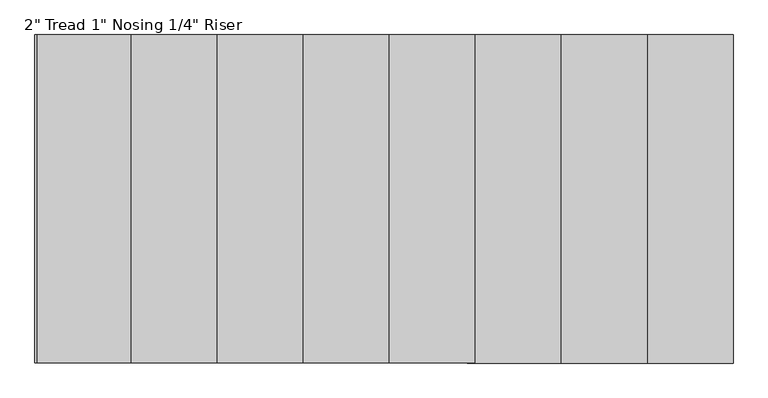
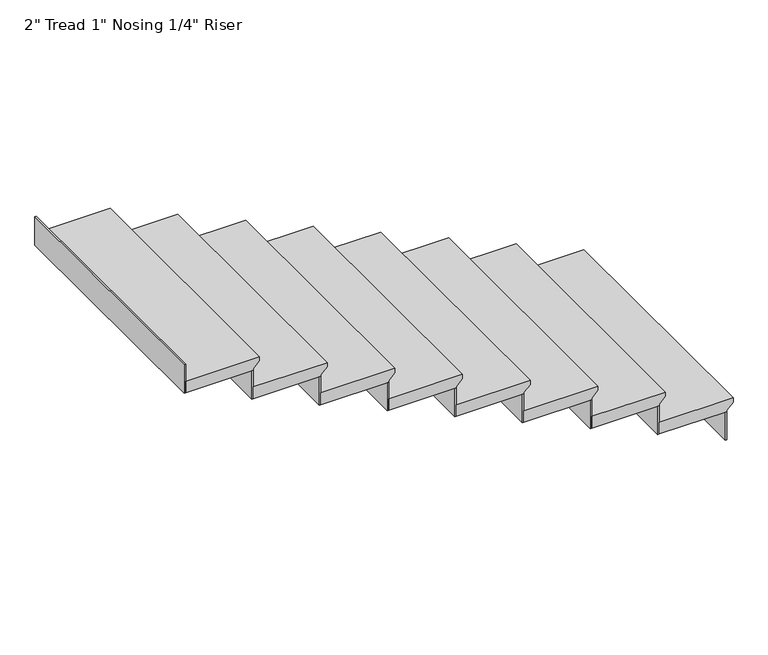
"""IFC4 building model written with IfcOpenShell, lengths in millimetres: stair flight geometry."""

import ifcopenshell
import ifcopenshell.guid

model = None  # the IFC model being written
_history = None  # IfcOwnerHistory: only IFC2X3 demands one
_inside = {}  # id of a spatial element -> (the spatial element, [elements in it])
_under = {}  # id of a project, library or spatial element -> (it, [spatial elements below it])
_declared = {}  # id of a project -> (the project, [libraries it declares])
_typed = {}  # id of a type object -> (the type object, [elements of that type])
_made_of = {}  # id of a material, layer set ... -> (it, [elements and type objects made of it])


def new_model(schema):
    """Start an empty IFC model of exactly this schema.

    Asked for "IFC4X3", IfcOpenShell would pick the latest addendum, in which some entities
    have other attributes; the version numbers below select the first issue.
    IFC2X3 requires an IfcOwnerHistory on every rooted entity: one is made here for all.
    """
    global model, _history
    if schema == "IFC4X3":
        model = ifcopenshell.file(schema_version=(4, 3, 0, 0))
    else:
        model = ifcopenshell.file(schema=schema)
    _inside.clear()
    _under.clear()
    _declared.clear()
    _typed.clear()
    _made_of.clear()
    _history = None
    if model.schema == "IFC2X3":
        org = make("IfcOrganization", Name="unknown")
        user = make(
            "IfcPersonAndOrganization",
            ThePerson=make("IfcPerson", FamilyName="unknown"),
            TheOrganization=org,
        )
        app = make(
            "IfcApplication",
            ApplicationDeveloper=org,
            Version="unknown",
            ApplicationFullName="unknown",
            ApplicationIdentifier="unknown",
        )
        _history = make(
            "IfcOwnerHistory",
            OwningUser=user,
            OwningApplication=app,
            ChangeAction="ADDED",
            CreationDate=0,
        )
    return model


def make(cls, **values):
    """One entity of the class cls with the attributes given. An attribute that is None is left unset."""
    return model.create_entity(
        cls, **{name: value for name, value in values.items() if value is not None}
    )


def rooted(cls, **values):
    """An entity with a GlobalId (a new one), such as an element, a storey or a relation."""
    return make(cls, GlobalId=ifcopenshell.guid.new(), OwnerHistory=_history, **values)


def si_unit(unit_type, name, prefix=None):
    """IfcSIUnit, for example si_unit("LENGTHUNIT", "METRE", prefix="MILLI")."""
    return make("IfcSIUnit", UnitType=unit_type, Prefix=prefix, Name=name)


def assignment(units):
    """IfcUnitAssignment: the units of a project."""
    return None if units is None else make("IfcUnitAssignment", Units=units)


def point(xyz):
    """IfcCartesianPoint."""
    return None if xyz is None else make("IfcCartesianPoint", Coordinates=xyz)


def direction(xyz):
    """IfcDirection."""
    return None if xyz is None else make("IfcDirection", DirectionRatios=xyz)


def frame(location, z_axis=None, x_axis=None):
    """IfcAxis2Placement3D, a coordinate frame: its origin and axes. An axis left out is left unset."""
    return make(
        "IfcAxis2Placement3D",
        Location=point(location),
        Axis=direction(z_axis),
        RefDirection=direction(x_axis),
    )


def origin():
    """The frame at (0, 0, 0) with its axes left unset."""
    return frame((0.0, 0.0, 0.0))


def place(relative_to, where):
    """IfcLocalPlacement: puts the frame where relative to a parent placement (None: the world)."""
    return make(
        "IfcLocalPlacement", PlacementRelTo=relative_to, RelativePlacement=where
    )


def context(
    kind, dimensions, precision=None, world=None, true_north=None, identifier=None
):
    """IfcGeometricRepresentationContext, for example the 3D "Model" context."""
    return make(
        "IfcGeometricRepresentationContext",
        ContextIdentifier=identifier,
        ContextType=kind,
        CoordinateSpaceDimension=dimensions,
        Precision=precision,
        WorldCoordinateSystem=world,
        TrueNorth=true_north,
    )


def project(units=None, contexts=None):
    """IfcProject with its units and contexts."""
    return rooted(
        "IfcProject",
        Name="project",
        RepresentationContexts=contexts,
        UnitsInContext=assignment(units),
    )


def spatial(cls, under=None, at=None, **own):
    """A site, building, storey or space (cls), placed at a placement, below another one or the project."""
    s = rooted(cls, ObjectPlacement=at, **own)
    if under is not None:
        _under.setdefault(under.id(), (under, []))[1].append(s)
    return s


def faces_of(points, faces, orient=None, outer=None):
    """IfcFace entities. A face is a list of loops; a loop is a list of indices into points, from 0.

    orient and outer hold one flag for each loop. By default every Orientation is true, the
    first loop of a face is its IfcFaceOuterBound and the others are IfcFaceBound.
    """
    made = []
    for i, loops in enumerate(faces):
        bounds = []
        for j, loop in enumerate(loops):
            is_outer = j == 0 if outer is None else outer[i][j]
            bounds.append(
                make(
                    "IfcFaceOuterBound" if is_outer else "IfcFaceBound",
                    Bound=make("IfcPolyLoop", Polygon=[points[k] for k in loop]),
                    Orientation=True if orient is None else orient[i][j],
                )
            )
        made.append(make("IfcFace", Bounds=bounds))
    return made


def faceted_brep(points, faces, orient=None, outer=None, voids=None):
    """IfcFacetedBrep: a solid bounded by flat faces; with voids (closed shells), ...WithVoids."""
    shared = [point(p) for p in points]
    hull = make("IfcClosedShell", CfsFaces=faces_of(shared, faces, orient, outer))
    if voids is None:
        return make("IfcFacetedBrep", Outer=hull)
    return make(
        "IfcFacetedBrepWithVoids",
        Outer=hull,
        Voids=[
            make(cls, CfsFaces=faces_of(shared, fs, o, b)) for cls, fs, o, b in voids
        ],
    )


def shape(context_of_items, identifier, shape_type, items):
    """IfcShapeRepresentation: the items that make up one representation, for example the "Body"."""
    return make(
        "IfcShapeRepresentation",
        ContextOfItems=context_of_items,
        RepresentationIdentifier=identifier,
        RepresentationType=shape_type,
        Items=items,
    )


def source(mapping_origin, context_of_items, identifier, shape_type, items):
    """IfcRepresentationMap: a shape defined once, which mapped items show again and again."""
    return make(
        "IfcRepresentationMap",
        MappingOrigin=mapping_origin,
        MappedRepresentation=shape(context_of_items, identifier, shape_type, items),
    )


def transform(
    local_origin,
    x_axis=None,
    y_axis=None,
    z_axis=None,
    scale=None,
    scale2=None,
    scale3=None,
    uniform=True,
):
    """IfcCartesianTransformationOperator3D, or its non-uniform kind. x_axis, y_axis, z_axis: its Axis1, 2, 3."""
    if uniform:
        return make(
            "IfcCartesianTransformationOperator3D",
            Axis1=direction(x_axis),
            Axis2=direction(y_axis),
            LocalOrigin=point(local_origin),
            Scale=scale,
            Axis3=direction(z_axis),
        )
    return make(
        "IfcCartesianTransformationOperator3DnonUniform",
        Axis1=direction(x_axis),
        Axis2=direction(y_axis),
        LocalOrigin=point(local_origin),
        Scale=scale,
        Axis3=direction(z_axis),
        Scale2=scale2,
        Scale3=scale3,
    )


def mapped(mapping_source, mapping_target):
    """IfcMappedItem: shows the shape of a source again, moved by a transform."""
    return make(
        "IfcMappedItem", MappingSource=mapping_source, MappingTarget=mapping_target
    )


def made_of(thing, what):
    """Note that an element or type object is made of a material, layer set ...; save() writes the relation."""
    if what is not None:
        _made_of.setdefault(what.id(), (what, []))[1].append(thing)
    return thing


def element(
    cls,
    number,
    at=None,
    inside=None,
    cuts=None,
    type_object=None,
    material=None,
    context=None,
    identifier="Body",
    shape_type=None,
    held_by="IfcProductDefinitionShape",
    body=None,
    shapes=None,
    **own,
):
    """One element of the class cls, such as IfcWall. Its Tag is "e" and its number.

    at: its placement. inside: the storey or other place that contains it. cuts: it is an
    opening in that element (IfcRelVoidsElement). A single representation is given by context,
    identifier, shape_type and body (its items); several are given by shapes. held_by: the class
    of the entity that holds the representations. save() writes the other relations.
    """
    e = rooted(cls, Tag="e%d" % number, ObjectPlacement=at, **own)
    if body is not None:
        shapes = [shape(context, identifier, shape_type, body)]
    if shapes is not None:
        e.Representation = make(held_by, Representations=shapes)
    if inside is not None:
        _inside.setdefault(inside.id(), (inside, []))[1].append(e)
    if cuts is not None:
        rooted(
            "IfcRelVoidsElement", RelatingBuildingElement=cuts, RelatedOpeningElement=e
        )
    if type_object is not None:
        _typed.setdefault(type_object.id(), (type_object, []))[1].append(e)
    return made_of(e, material)


def aggregate(whole, parts):
    """IfcRelAggregates: a whole, such as a stair, and the parts it consists of."""
    return rooted("IfcRelAggregates", RelatingObject=whole, RelatedObjects=parts)


def save(model, path):
    """Write the relations noted so far, then the file.

    IfcRelAggregates (storeys below a building ...), IfcRelContainedInSpatialStructure (elements
    in a storey), IfcRelDefinesByType, IfcRelAssociatesMaterial and IfcRelDeclares: one each for
    every whole, place, type object, material and project.
    """
    for whole, parts in _under.values():
        aggregate(whole, parts)
    for where, things in _inside.values():
        rooted(
            "IfcRelContainedInSpatialStructure",
            RelatedElements=things,
            RelatingStructure=where,
        )
    for kind, things in _typed.values():
        rooted("IfcRelDefinesByType", RelatedObjects=things, RelatingType=kind)
    for what, things in _made_of.values():
        rooted("IfcRelAssociatesMaterial", RelatedObjects=things, RelatingMaterial=what)
    for by, libraries in _declared.values():
        rooted("IfcRelDeclares", RelatingContext=by, RelatedDefinitions=libraries)
    model.write(path)


def stair_flight_a08092b1(model_context):
    return source(origin(), model_context, "Body", "Brep", [
        faceted_brep([(665956.388677, -549416.0413841, 1216.6256757), (665956.388677, -549416.0413841, 1235.6756757), (665956.388677, -550482.8413841, 1235.6756757), (665956.388677, -550482.8413841, 1216.6256757), (665930.988677, -549416.0413841, 1191.2256757), (665930.988677, -550482.8413841, 1191.2256757), (665651.588677, -549416.0413841, 1235.6756757), (665651.588677, -550482.8413841, 1235.6756757), (665930.988677, -550482.8413841, 1184.8756757), (665651.588677, -550482.8413841, 1184.8756757), (665651.588677, -549416.0413841, 1184.8756757), (665930.988677, -549416.0413841, 1184.8756757)], [[[0, 1, 2, 3]], [[4, 0, 3, 5]], [[2, 1, 6, 7]], [[8, 9, 10, 11]], [[2, 7, 9, 8, 5, 3]], [[8, 11, 4, 5]], [[6, 1, 0, 4, 11, 10]], [[7, 6, 10, 9]]]),
        faceted_brep([(665930.988677, -549416.0413841, 1184.8756757), (665930.988677, -549416.0413841, 1061.3081081), (665924.638677, -549416.0413841, 1061.3081081), (665924.638677, -549416.0413841, 1184.8756757), (665930.988677, -550482.8413841, 1184.8756757), (665924.638677, -550482.8413841, 1184.8756757), (665924.638677, -550482.8413841, 1061.3081081), (665930.988677, -550482.8413841, 1061.3081081)], [[[0, 1, 2, 3]], [[4, 5, 6, 7]], [[1, 0, 4, 7]], [[2, 1, 7, 6]], [[3, 2, 6, 5]], [[0, 3, 5, 4]]]),
        faceted_brep([(665651.588677, -549416.0413841, 1308.4432432), (665651.588677, -549416.0413841, 1184.8756757), (665645.238677, -549416.0413841, 1184.8756757), (665645.238677, -549416.0413841, 1308.4432432), (665651.588677, -550482.8413841, 1308.4432432), (665645.238677, -550482.8413841, 1308.4432432), (665645.238677, -550482.8413841, 1184.8756757), (665651.588677, -550482.8413841, 1184.8756757)], [[[0, 1, 2, 3]], [[4, 5, 6, 7]], [[1, 0, 4, 7]], [[2, 1, 7, 6]], [[3, 2, 6, 5]], [[0, 3, 5, 4]]]),
        faceted_brep([(665676.988677, -550482.8413841, 1359.2432432), (665676.988677, -549416.0413841, 1359.2432432), (665372.188677, -549416.0413841, 1359.2432432), (665372.188677, -550482.8413841, 1359.2432432), (665651.588677, -550482.8413841, 1308.4432432), (665372.188677, -550482.8413841, 1308.4432432), (665372.188677, -549416.0413841, 1308.4432432), (665651.588677, -549416.0413841, 1308.4432432), (665651.588677, -550482.8413841, 1314.7932432), (665676.988677, -550482.8413841, 1340.1932432), (665651.588677, -549416.0413841, 1314.7932432), (665676.988677, -549416.0413841, 1340.1932432)], [[[0, 1, 2, 3]], [[4, 5, 6, 7]], [[0, 3, 5, 4, 8, 9]], [[4, 7, 10, 8]], [[2, 1, 11, 10, 7, 6]], [[3, 2, 6, 5]], [[11, 1, 0, 9]], [[10, 11, 9, 8]]]),
        faceted_brep([(665372.188677, -549416.0413841, 1432.0108108), (665372.188677, -549416.0413841, 1308.4432432), (665365.838677, -549416.0413841, 1308.4432432), (665365.838677, -549416.0413841, 1432.0108108), (665372.188677, -550482.8413841, 1432.0108108), (665365.838677, -550482.8413841, 1432.0108108), (665365.838677, -550482.8413841, 1308.4432432), (665372.188677, -550482.8413841, 1308.4432432)], [[[0, 1, 2, 3]], [[4, 5, 6, 7]], [[1, 0, 4, 7]], [[2, 1, 7, 6]], [[3, 2, 6, 5]], [[0, 3, 5, 4]]]),
        faceted_brep([(665397.588677, -550482.8413841, 1482.8108108), (665397.588677, -549416.0413841, 1482.8108108), (665092.788677, -549416.0413841, 1482.8108108), (665092.788677, -550482.8413841, 1482.8108108), (665372.188677, -550482.8413841, 1432.0108108), (665092.788677, -550482.8413841, 1432.0108108), (665092.788677, -549416.0413841, 1432.0108108), (665372.188677, -549416.0413841, 1432.0108108), (665372.188677, -550482.8413841, 1438.3608108), (665397.588677, -550482.8413841, 1463.7608108), (665372.188677, -549416.0413841, 1438.3608108), (665397.588677, -549416.0413841, 1463.7608108)], [[[0, 1, 2, 3]], [[4, 5, 6, 7]], [[0, 3, 5, 4, 8, 9]], [[4, 7, 10, 8]], [[2, 1, 11, 10, 7, 6]], [[3, 2, 6, 5]], [[11, 1, 0, 9]], [[10, 11, 9, 8]]]),
        faceted_brep([(665092.788677, -549416.0413841, 1555.5783784), (665092.788677, -549416.0413841, 1432.0108108), (665086.438677, -549416.0413841, 1432.0108108), (665086.438677, -549416.0413841, 1555.5783784), (665092.788677, -550482.8413841, 1555.5783784), (665086.438677, -550482.8413841, 1555.5783784), (665086.438677, -550482.8413841, 1432.0108108), (665092.788677, -550482.8413841, 1432.0108108)], [[[0, 1, 2, 3]], [[4, 5, 6, 7]], [[1, 0, 4, 7]], [[2, 1, 7, 6]], [[3, 2, 6, 5]], [[0, 3, 5, 4]]]),
        faceted_brep([(665118.188677, -550482.8413841, 1606.3783784), (665118.188677, -549416.0413841, 1606.3783784), (664813.388677, -549416.0413841, 1606.3783784), (664813.388677, -550482.8413841, 1606.3783784), (665092.788677, -550482.8413841, 1555.5783784), (664813.388677, -550482.8413841, 1555.5783784), (664813.388677, -549416.0413841, 1555.5783784), (665092.788677, -549416.0413841, 1555.5783784), (665092.788677, -550482.8413841, 1561.9283784), (665118.188677, -550482.8413841, 1587.3283784), (665092.788677, -549416.0413841, 1561.9283784), (665118.188677, -549416.0413841, 1587.3283784)], [[[0, 1, 2, 3]], [[4, 5, 6, 7]], [[0, 3, 5, 4, 8, 9]], [[4, 7, 10, 8]], [[2, 1, 11, 10, 7, 6]], [[3, 2, 6, 5]], [[11, 1, 0, 9]], [[10, 11, 9, 8]]]),
        faceted_brep([(664813.388677, -549416.0413841, 1679.1459459), (664813.388677, -549416.0413841, 1555.5783784), (664807.038677, -549416.0413841, 1555.5783784), (664807.038677, -549416.0413841, 1679.1459459), (664813.388677, -550482.8413841, 1679.1459459), (664807.038677, -550482.8413841, 1679.1459459), (664807.038677, -550482.8413841, 1555.5783784), (664813.388677, -550482.8413841, 1555.5783784)], [[[0, 1, 2, 3]], [[4, 5, 6, 7]], [[1, 0, 4, 7]], [[2, 1, 7, 6]], [[3, 2, 6, 5]], [[0, 3, 5, 4]]]),
        faceted_brep([(664838.788677, -550482.8413841, 1729.9459459), (664838.788677, -549416.0413841, 1729.9459459), (664533.988677, -549416.0413841, 1729.9459459), (664533.988677, -550482.8413841, 1729.9459459), (664813.388677, -550482.8413841, 1679.1459459), (664533.988677, -550482.8413841, 1679.1459459), (664533.988677, -549416.0413841, 1679.1459459), (664813.388677, -549416.0413841, 1679.1459459), (664813.388677, -550482.8413841, 1685.4959459), (664838.788677, -550482.8413841, 1710.8959459), (664813.388677, -549416.0413841, 1685.4959459), (664838.788677, -549416.0413841, 1710.8959459)], [[[0, 1, 2, 3]], [[4, 5, 6, 7]], [[0, 3, 5, 4, 8, 9]], [[4, 7, 10, 8]], [[2, 1, 11, 10, 7, 6]], [[3, 2, 6, 5]], [[11, 1, 0, 9]], [[10, 11, 9, 8]]]),
        faceted_brep([(664533.988677, -549416.0413841, 1802.7135135), (664533.988677, -549416.0413841, 1679.1459459), (664527.638677, -549416.0413841, 1679.1459459), (664527.638677, -549416.0413841, 1802.7135135), (664533.988677, -550482.8413841, 1802.7135135), (664527.638677, -550482.8413841, 1802.7135135), (664527.638677, -550482.8413841, 1679.1459459), (664533.988677, -550482.8413841, 1679.1459459)], [[[0, 1, 2, 3]], [[4, 5, 6, 7]], [[1, 0, 4, 7]], [[2, 1, 7, 6]], [[3, 2, 6, 5]], [[0, 3, 5, 4]]]),
        faceted_brep([(664559.388677, -550482.8413841, 1853.5135135), (664559.388677, -549416.0413841, 1853.5135135), (664254.588677, -549416.0413841, 1853.5135135), (664254.588677, -550482.8413841, 1853.5135135), (664533.988677, -550482.8413841, 1802.7135135), (664254.588677, -550482.8413841, 1802.7135135), (664254.588677, -549416.0413841, 1802.7135135), (664533.988677, -549416.0413841, 1802.7135135), (664533.988677, -550482.8413841, 1809.0635135), (664559.388677, -550482.8413841, 1834.4635135), (664533.988677, -549416.0413841, 1809.0635135), (664559.388677, -549416.0413841, 1834.4635135)], [[[0, 1, 2, 3]], [[4, 5, 6, 7]], [[0, 3, 5, 4, 8, 9]], [[4, 7, 10, 8]], [[2, 1, 11, 10, 7, 6]], [[3, 2, 6, 5]], [[11, 1, 0, 9]], [[10, 11, 9, 8]]]),
        faceted_brep([(664254.588677, -549416.0413841, 1926.2810811), (664254.588677, -549416.0413841, 1802.7135135), (664248.238677, -549416.0413841, 1802.7135135), (664248.238677, -549416.0413841, 1926.2810811), (664254.588677, -550482.8413841, 1926.2810811), (664248.238677, -550482.8413841, 1926.2810811), (664248.238677, -550482.8413841, 1802.7135135), (664254.588677, -550482.8413841, 1802.7135135)], [[[0, 1, 2, 3]], [[4, 5, 6, 7]], [[1, 0, 4, 7]], [[2, 1, 7, 6]], [[3, 2, 6, 5]], [[0, 3, 5, 4]]]),
        faceted_brep([(664279.988677, -550482.8413841, 1977.0810811), (664279.988677, -549416.0413841, 1977.0810811), (663975.188677, -549416.0413841, 1977.0810811), (663975.188677, -550482.8413841, 1977.0810811), (664254.588677, -550482.8413841, 1926.2810811), (663975.188677, -550482.8413841, 1926.2810811), (663975.188677, -549416.0413841, 1926.2810811), (664254.588677, -549416.0413841, 1926.2810811), (664254.588677, -550482.8413841, 1932.6310811), (664279.988677, -550482.8413841, 1958.0310811), (664254.588677, -549416.0413841, 1932.6310811), (664279.988677, -549416.0413841, 1958.0310811)], [[[0, 1, 2, 3]], [[4, 5, 6, 7]], [[0, 3, 5, 4, 8, 9]], [[4, 7, 10, 8]], [[2, 1, 11, 10, 7, 6]], [[3, 2, 6, 5]], [[11, 1, 0, 9]], [[10, 11, 9, 8]]]),
        faceted_brep([(663695.788677, -549416.0413841, 2173.4162162), (663695.788677, -549416.0413841, 2049.8486486), (663689.438677, -549416.0413841, 2049.8486486), (663689.438677, -549416.0413841, 2173.4162162), (663695.788677, -550482.8413841, 2173.4162162), (663689.438677, -550482.8413841, 2173.4162162), (663689.438677, -550482.8413841, 2049.8486486), (663695.788677, -550482.8413841, 2049.8486486)], [[[0, 1, 2, 3]], [[4, 5, 6, 7]], [[1, 0, 4, 7]], [[2, 1, 7, 6]], [[3, 2, 6, 5]], [[0, 3, 5, 4]]]),
        faceted_brep([(663975.188677, -549416.0413841, 2049.8486486), (663975.188677, -549416.0413841, 1926.2810811), (663968.838677, -549416.0413841, 1926.2810811), (663968.838677, -549416.0413841, 2049.8486486), (663975.188677, -550482.8413841, 2049.8486486), (663968.838677, -550482.8413841, 2049.8486486), (663968.838677, -550482.8413841, 1926.2810811), (663975.188677, -550482.8413841, 1926.2810811)], [[[0, 1, 2, 3]], [[4, 5, 6, 7]], [[1, 0, 4, 7]], [[2, 1, 7, 6]], [[3, 2, 6, 5]], [[0, 3, 5, 4]]]),
        faceted_brep([(664000.588677, -550482.8413841, 2100.6486486), (664000.588677, -549416.0413841, 2100.6486486), (663721.188677, -549416.0413841, 2100.6486486), (663695.788677, -549416.0413841, 2100.6486486), (663695.788677, -550482.8413841, 2100.6486486), (663975.188677, -550482.8413841, 2049.8486486), (663695.788677, -550482.8413841, 2049.8486486), (663695.788677, -549416.0413841, 2049.8486486), (663721.188677, -549416.0413841, 2049.8486486), (663975.188677, -549416.0413841, 2049.8486486), (663975.188677, -550482.8413841, 2056.1986486), (664000.588677, -550482.8413841, 2081.5986486), (663975.188677, -549416.0413841, 2056.1986486), (664000.588677, -549416.0413841, 2081.5986486)], [[[0, 1, 2, 3, 4]], [[5, 6, 7, 8, 9]], [[0, 4, 6, 5, 10, 11]], [[5, 9, 12, 10]], [[2, 1, 13, 12, 9, 8]], [[3, 2, 8, 7]], [[4, 3, 7, 6]], [[13, 1, 0, 11]], [[12, 13, 11, 10]]]),
    ])


if __name__ == "__main__":
    model = new_model("IFC4")
    model_context = context("Model", 3, world=origin())
    ifc_project = project(units=[si_unit("LENGTHUNIT", "METRE", prefix="MILLI")], contexts=[model_context])
    site = spatial("IfcSite", under=ifc_project)
    building = spatial("IfcBuilding", under=site)
    placement = place(None, origin())
    stair_flight_shape = stair_flight_a08092b1(model_context)
    element("IfcStairFlight", 1, ObjectType="2\" Tread 1\" Nosing 1/4\" Riser", at=placement, inside=building, context=model_context, shape_type="MappedRepresentation", body=[
        mapped(stair_flight_shape, transform((0.0, 0.0, 0.0), x_axis=(1.0, 0.0, 0.0), y_axis=(0.0, 1.0, 0.0), z_axis=(0.0, 0.0, 1.0))),
    ])
    save(model, "model.ifc")
